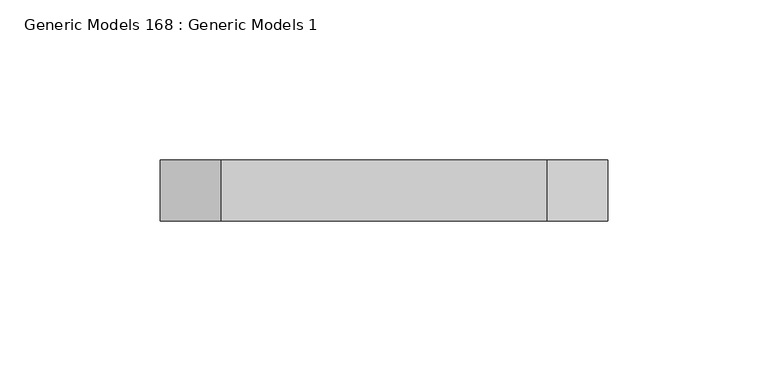
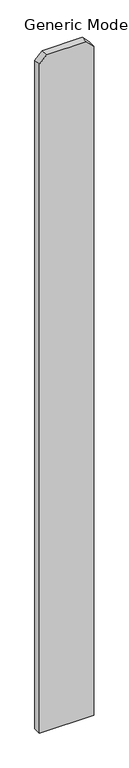
"""IFC4 building model written with IfcOpenShell, lengths in millimetres: proxy geometry, Generic Models 168 : Generic Models 1."""

from ifc_helpers import new_model, si_unit, frame, origin, place, context, project, spatial, polyline, outline, extrude, source, transform, mapped, element, save


def generic_models_168_generic_models_1_c133e3c9(model_context):
    return source(origin(), model_context, "Body", "SweptSolid", [
        extrude(outline(polyline([(76.2, 55599.0125), (1885.95, 55599.0125), (1905.0, 55579.9625), (1905.0, 55478.3625), (1885.95, 55459.3125), (76.2, 55459.3125), (76.2, 55599.0125)])), frame((0.0, 547.6875, 0.0), z_axis=(0.0, 1.0, 0.0), x_axis=(0.0, 0.0, 1.0)), (0.0, 0.0, 1.0), 19.05),
    ])


if __name__ == "__main__":
    model = new_model("IFC4")
    model_context = context("Model", 3, world=origin())
    ifc_project = project(units=[si_unit("LENGTHUNIT", "METRE", prefix="MILLI")], contexts=[model_context])
    site = spatial("IfcSite", under=ifc_project)
    building = spatial("IfcBuilding", under=site)
    placement = place(None, origin())
    generic_models_168_generic_models_1_shape = generic_models_168_generic_models_1_c133e3c9(model_context)
    element("IfcBuildingElementProxy", 1, Name="Generic Models 168 : Generic Models 1", ObjectType="Generic Models 168 : Generic Models 1", at=placement, inside=building, context=model_context, shape_type="MappedRepresentation", body=[
        mapped(generic_models_168_generic_models_1_shape, transform((0.0, 0.0, 0.0), x_axis=(1.0, 0.0, 0.0), y_axis=(0.0, 1.0, 0.0), z_axis=(0.0, 0.0, 1.0))),
    ])
    save(model, "model.ifc")

# Revit data of these elements
# Element 1 (IfcBuildingElementProxy, "Generic Models 168 : Generic Models 1")
#   Materials on its faces: "VERTICAL 1X6 CEDAR PLANKS W/ CLEAR WOOD SEALER"
# Materials
#   "VERTICAL 1X6 CEDAR PLANKS W/ CLEAR WOOD SEALER": class "Wood", colour RGB 234 198 147, transparency 0, Description = "Pinus Echinata", Cost = 0
